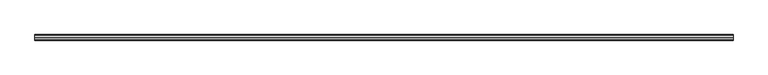
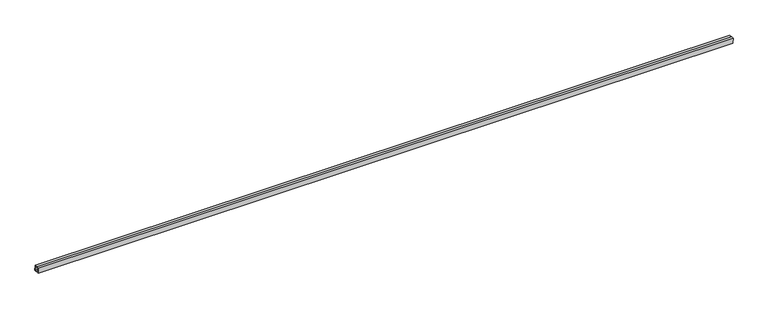
"""IFC4 building model written with IfcOpenShell, lengths in millimetres: proxy geometry, Inner panel:Inner panel:1:Inner panel:1 : Inner panel:Inner panel:300324:2:Inner panel:1:Inner panel:1 : Inner panel:Inner panel:300324:2 : Inner panel:Inner panel:1:Inner panel:1 : Inner panel:Inner panel:300324:300043:55 : Inner panel:Inner panel:1:Inner panel:1 : Inner panel:Inner panel:300324:2:Inner panel:1:Inner panel:1 : Inner panel:Inner panel:300324:2 : Inner panel:Inner panel:1:Inner panel:1 : Inner panel:Inner panel:300324:300043:308120."""

from ifc_helpers import new_model, si_unit, frame, origin, place, context, project, spatial, polyline, outline, extrude, source, transform, mapped, element, save


def generic_models_662411af(model_context):
    return source(origin(), model_context, "Body", "SweptSolid", [
        extrude(outline(polyline([(-578476.5317668, 3971.7383355), (-578458.2913437, 3972.4983531), (-578456.7052199, 3934.431383), (-578494.77219, 3932.8452593), (-578496.3583138, 3970.9122294), (-578478.1178906, 3971.672247), (-578478.0187579, 3969.2930614), (-578493.8799954, 3968.6321765), (-578492.4921371, 3935.3235776), (-578459.1835383, 3936.7114359), (-578460.5713966, 3970.0200347), (-578476.4326341, 3969.3591498), (-578476.5317668, 3971.7383355)])), frame((659327.2367238, 0.0, 0.0), z_axis=(1.0, 0.0, 0.0), x_axis=(0.0, 1.0, 0.0)), (0.0, 0.0, 1.0), 4876.8),
    ])


if __name__ == "__main__":
    model = new_model("IFC4")
    model_context = context("Model", 3, world=origin())
    ifc_project = project(units=[si_unit("LENGTHUNIT", "METRE", prefix="MILLI")], contexts=[model_context])
    site = spatial("IfcSite", under=ifc_project)
    building = spatial("IfcBuilding", under=site)
    placement = place(None, origin())
    generic_models_shape = generic_models_662411af(model_context)
    element("IfcBuildingElementProxy", 1, Name="Inner panel:Inner panel:1:Inner panel:1 : Inner panel:Inner panel:300324:2:Inner panel:1:Inner panel:1 : Inner panel:Inner panel:300324:2 : Inner panel:Inner panel:1:Inner panel:1 : Inner panel:Inner panel:300324:300043:55 : Inner panel:Inner panel:1:Inner panel:1 : Inner panel:Inner panel:300324:2:Inner panel:1:Inner panel:1 : Inner panel:Inner panel:300324:2 : Inner panel:Inner panel:1:Inner panel:1 : Inner panel:Inner panel:300324:300043:308120", ObjectType="Inner panel:Inner panel:1:Inner panel:1 : Inner panel:Inner panel:300324:2:Inner panel:1:Inner panel:1 : Inner panel:Inner panel:300324:2 : Inner panel:Inner panel:1:Inner panel:1 : Inner panel:Inner panel:300324:300043:55 : Inner panel:Inner panel:1:Inner panel:1 : Inner panel:Inner panel:300324:2:Inner panel:1:Inner panel:1 : Inner panel:Inner panel:300324:2 : Inner panel:Inner panel:1:Inner panel:1 : Inner panel:Inner panel:300324:300043:308120", at=placement, inside=building, context=model_context, shape_type="MappedRepresentation", body=[
        mapped(generic_models_shape, transform((0.0, 0.0, 0.0), x_axis=(1.0, 0.0, 0.0), y_axis=(0.0, 1.0, 0.0), z_axis=(0.0, 0.0, 1.0))),
    ])
    save(model, "model.ifc")

# Revit data of these elements
# Type "Inner panel:Inner panel:1:Inner panel:1 : Inner panel:Inner panel:300324:2:Inner panel:1:Inner panel:1 : Inner panel:Inner panel:300324:2 : Inner panel:Inner panel:1:Inner panel:1 : Inner panel:Inner panel:300324:300043:55 : Inner panel:Inner panel:1:Inner panel:1 : Inner panel:Inner panel:300324:2:Inner panel:1:Inner panel:1 : Inner panel:Inner panel:300324:2 : Inner panel:Inner panel:1:Inner panel:1 : Inner panel:Inner panel:300324:300043:308120"
#   NameOverride = "Inner panel:Inner panel:1:Inner panel:1 : Inner panel:Inner panel:300324:2:Inner panel:1:Inner panel:1 : Inner panel:Inner panel:300324:2 : Inner panel:Inner panel:1:Inner panel:1 : Inner panel:Inner panel:300324:300043:308120"
#   ObjectTypeOverride = "Inner panel:1:Inner panel:1 : Inner panel:Inner panel:300324:2 : Inner panel:Inner panel:1:Inner panel:1 : Inner panel:Inner panel:300324:300043"
#   Reference = "Inner panel"
#   Tag = "308120"
# Element 1 (IfcBuildingElementProxy, "Inner panel:Inner panel:1:Inner panel:1 : Inner panel:Inner panel:300324:2:Inner panel:1:Inner panel:1 : Inner panel:Inner panel:300324:2 : Inner panel:Inner panel:1:Inner panel:1 : Inner panel:Inner panel:300324:300043:55 : Inner panel:Inner panel:1:Inner panel:1 : Inner panel:Inner panel:300324:2:Inner panel:1:Inner panel:1 : Inner panel:Inner panel:300324:2 : Inner panel:Inner panel:1:Inner panel:1 : Inner panel:Inner panel:300324:300043:308120")
#   Materials on its faces: "1 1/2\" X 1 1/2\" SPLIT-SEAM SQUARE TUBING (~24\" CANTILEVER FROM C.L. OF GLULAM)"
# Materials
#   "1 1/2\" X 1 1/2\" SPLIT-SEAM SQUARE TUBING (~24\" CANTILEVER FROM C.L. OF GLULAM)": class "Unassigned", colour RGB 202 201 200, transparency 0, Cost = 0
